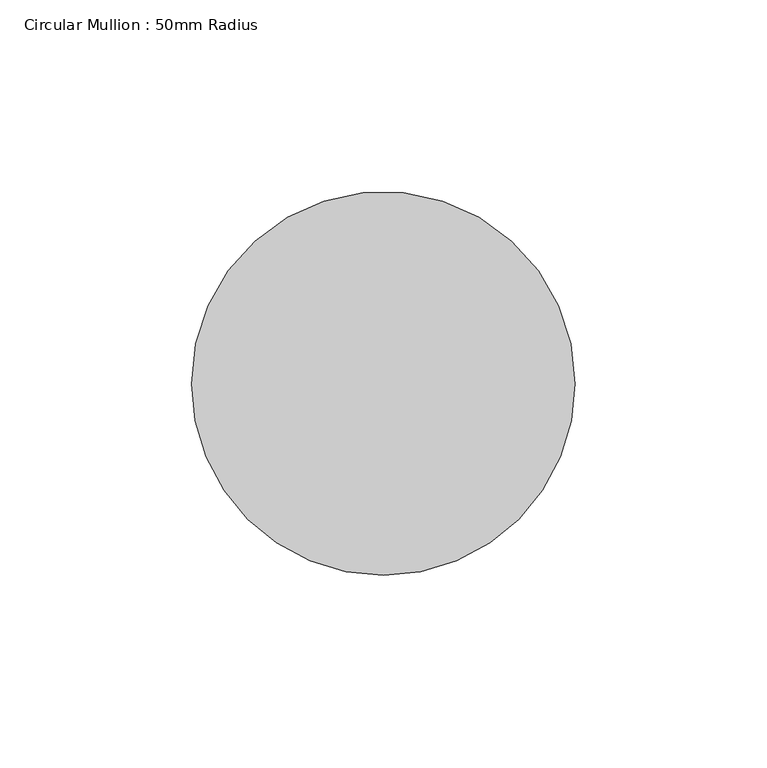
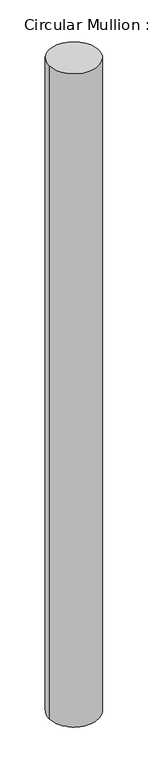
"""IFC4 building model written with IfcOpenShell, lengths in millimetres: member geometry, Circular Mullion : 50mm Radius."""

import ifcopenshell
import ifcopenshell.guid

model = None  # the IFC model being written
_history = None  # IfcOwnerHistory: only IFC2X3 demands one
_inside = {}  # id of a spatial element -> (the spatial element, [elements in it])
_under = {}  # id of a project, library or spatial element -> (it, [spatial elements below it])
_declared = {}  # id of a project -> (the project, [libraries it declares])
_typed = {}  # id of a type object -> (the type object, [elements of that type])
_made_of = {}  # id of a material, layer set ... -> (it, [elements and type objects made of it])


def new_model(schema):
    """Start an empty IFC model of exactly this schema.

    Asked for "IFC4X3", IfcOpenShell would pick the latest addendum, in which some entities
    have other attributes; the version numbers below select the first issue.
    IFC2X3 requires an IfcOwnerHistory on every rooted entity: one is made here for all.
    """
    global model, _history
    if schema == "IFC4X3":
        model = ifcopenshell.file(schema_version=(4, 3, 0, 0))
    else:
        model = ifcopenshell.file(schema=schema)
    _inside.clear()
    _under.clear()
    _declared.clear()
    _typed.clear()
    _made_of.clear()
    _history = None
    if model.schema == "IFC2X3":
        org = make("IfcOrganization", Name="unknown")
        user = make(
            "IfcPersonAndOrganization",
            ThePerson=make("IfcPerson", FamilyName="unknown"),
            TheOrganization=org,
        )
        app = make(
            "IfcApplication",
            ApplicationDeveloper=org,
            Version="unknown",
            ApplicationFullName="unknown",
            ApplicationIdentifier="unknown",
        )
        _history = make(
            "IfcOwnerHistory",
            OwningUser=user,
            OwningApplication=app,
            ChangeAction="ADDED",
            CreationDate=0,
        )
    return model


def make(cls, **values):
    """One entity of the class cls with the attributes given. An attribute that is None is left unset."""
    return model.create_entity(
        cls, **{name: value for name, value in values.items() if value is not None}
    )


def rooted(cls, **values):
    """An entity with a GlobalId (a new one), such as an element, a storey or a relation."""
    return make(cls, GlobalId=ifcopenshell.guid.new(), OwnerHistory=_history, **values)


def si_unit(unit_type, name, prefix=None):
    """IfcSIUnit, for example si_unit("LENGTHUNIT", "METRE", prefix="MILLI")."""
    return make("IfcSIUnit", UnitType=unit_type, Prefix=prefix, Name=name)


def assignment(units):
    """IfcUnitAssignment: the units of a project."""
    return None if units is None else make("IfcUnitAssignment", Units=units)


def point(xyz):
    """IfcCartesianPoint."""
    return None if xyz is None else make("IfcCartesianPoint", Coordinates=xyz)


def direction(xyz):
    """IfcDirection."""
    return None if xyz is None else make("IfcDirection", DirectionRatios=xyz)


def frame(location, z_axis=None, x_axis=None):
    """IfcAxis2Placement3D, a coordinate frame: its origin and axes. An axis left out is left unset."""
    return make(
        "IfcAxis2Placement3D",
        Location=point(location),
        Axis=direction(z_axis),
        RefDirection=direction(x_axis),
    )


def origin():
    """The frame at (0, 0, 0) with its axes left unset."""
    return frame((0.0, 0.0, 0.0))


def place(relative_to, where):
    """IfcLocalPlacement: puts the frame where relative to a parent placement (None: the world)."""
    return make(
        "IfcLocalPlacement", PlacementRelTo=relative_to, RelativePlacement=where
    )


def context(
    kind, dimensions, precision=None, world=None, true_north=None, identifier=None
):
    """IfcGeometricRepresentationContext, for example the 3D "Model" context."""
    return make(
        "IfcGeometricRepresentationContext",
        ContextIdentifier=identifier,
        ContextType=kind,
        CoordinateSpaceDimension=dimensions,
        Precision=precision,
        WorldCoordinateSystem=world,
        TrueNorth=true_north,
    )


def project(units=None, contexts=None):
    """IfcProject with its units and contexts."""
    return rooted(
        "IfcProject",
        Name="project",
        RepresentationContexts=contexts,
        UnitsInContext=assignment(units),
    )


def spatial(cls, under=None, at=None, **own):
    """A site, building, storey or space (cls), placed at a placement, below another one or the project."""
    s = rooted(cls, ObjectPlacement=at, **own)
    if under is not None:
        _under.setdefault(under.id(), (under, []))[1].append(s)
    return s


def ellipse_curve(where, semi_axis1, semi_axis2):
    """IfcEllipse in the frame where."""
    return make(
        "IfcEllipse", Position=where, SemiAxis1=semi_axis1, SemiAxis2=semi_axis2
    )


def shape(context_of_items, identifier, shape_type, items):
    """IfcShapeRepresentation: the items that make up one representation, for example the "Body"."""
    return make(
        "IfcShapeRepresentation",
        ContextOfItems=context_of_items,
        RepresentationIdentifier=identifier,
        RepresentationType=shape_type,
        Items=items,
    )


def source(mapping_origin, context_of_items, identifier, shape_type, items):
    """IfcRepresentationMap: a shape defined once, which mapped items show again and again."""
    return make(
        "IfcRepresentationMap",
        MappingOrigin=mapping_origin,
        MappedRepresentation=shape(context_of_items, identifier, shape_type, items),
    )


def transform(
    local_origin,
    x_axis=None,
    y_axis=None,
    z_axis=None,
    scale=None,
    scale2=None,
    scale3=None,
    uniform=True,
):
    """IfcCartesianTransformationOperator3D, or its non-uniform kind. x_axis, y_axis, z_axis: its Axis1, 2, 3."""
    if uniform:
        return make(
            "IfcCartesianTransformationOperator3D",
            Axis1=direction(x_axis),
            Axis2=direction(y_axis),
            LocalOrigin=point(local_origin),
            Scale=scale,
            Axis3=direction(z_axis),
        )
    return make(
        "IfcCartesianTransformationOperator3DnonUniform",
        Axis1=direction(x_axis),
        Axis2=direction(y_axis),
        LocalOrigin=point(local_origin),
        Scale=scale,
        Axis3=direction(z_axis),
        Scale2=scale2,
        Scale3=scale3,
    )


def mapped(mapping_source, mapping_target):
    """IfcMappedItem: shows the shape of a source again, moved by a transform."""
    return make(
        "IfcMappedItem", MappingSource=mapping_source, MappingTarget=mapping_target
    )


def made_of(thing, what):
    """Note that an element or type object is made of a material, layer set ...; save() writes the relation."""
    if what is not None:
        _made_of.setdefault(what.id(), (what, []))[1].append(thing)
    return thing


def element(
    cls,
    number,
    at=None,
    inside=None,
    cuts=None,
    type_object=None,
    material=None,
    context=None,
    identifier="Body",
    shape_type=None,
    held_by="IfcProductDefinitionShape",
    body=None,
    shapes=None,
    **own,
):
    """One element of the class cls, such as IfcWall. Its Tag is "e" and its number.

    at: its placement. inside: the storey or other place that contains it. cuts: it is an
    opening in that element (IfcRelVoidsElement). A single representation is given by context,
    identifier, shape_type and body (its items); several are given by shapes. held_by: the class
    of the entity that holds the representations. save() writes the other relations.
    """
    e = rooted(cls, Tag="e%d" % number, ObjectPlacement=at, **own)
    if body is not None:
        shapes = [shape(context, identifier, shape_type, body)]
    if shapes is not None:
        e.Representation = make(held_by, Representations=shapes)
    if inside is not None:
        _inside.setdefault(inside.id(), (inside, []))[1].append(e)
    if cuts is not None:
        rooted(
            "IfcRelVoidsElement", RelatingBuildingElement=cuts, RelatedOpeningElement=e
        )
    if type_object is not None:
        _typed.setdefault(type_object.id(), (type_object, []))[1].append(e)
    return made_of(e, material)


def aggregate(whole, parts):
    """IfcRelAggregates: a whole, such as a stair, and the parts it consists of."""
    return rooted("IfcRelAggregates", RelatingObject=whole, RelatedObjects=parts)


def save(model, path):
    """Write the relations noted so far, then the file.

    IfcRelAggregates (storeys below a building ...), IfcRelContainedInSpatialStructure (elements
    in a storey), IfcRelDefinesByType, IfcRelAssociatesMaterial and IfcRelDeclares: one each for
    every whole, place, type object, material and project.
    """
    for whole, parts in _under.values():
        aggregate(whole, parts)
    for where, things in _inside.values():
        rooted(
            "IfcRelContainedInSpatialStructure",
            RelatedElements=things,
            RelatingStructure=where,
        )
    for kind, things in _typed.values():
        rooted("IfcRelDefinesByType", RelatedObjects=things, RelatingType=kind)
    for what, things in _made_of.values():
        rooted("IfcRelAssociatesMaterial", RelatedObjects=things, RelatingMaterial=what)
    for by, libraries in _declared.values():
        rooted("IfcRelDeclares", RelatingContext=by, RelatedDefinitions=libraries)
    model.write(path)


def plane_surface(at):
    """IfcPlane: the flat surface through the origin of the frame at, square to its z axis."""
    return make("IfcPlane", Position=at)


def cylinder_surface(at, radius):
    """IfcCylindricalSurface: all points at the distance radius from the z axis of the frame at."""
    return make("IfcCylindricalSurface", Position=at, Radius=radius)


def advanced_brep(points, edges, surfaces, faces):
    """IfcAdvancedBrep: a solid bounded by faces that lie on surfaces and meet in shared edges.

    An edge is (start, end): straight between two places in points (the first is 0);
    or (start, end, curve); or (start, end, curve, False) where it runs against its curve.
    A face is (place in surfaces, loops), or (place, loops, False) where it looks against
    its surface's normal. A loop lists edges by number (the first is 1), with a minus sign
    where the edge is run from its end to its start. The first loop is the outer one.
    """
    corners = [point(p) for p in points]
    vertices = [make("IfcVertexPoint", VertexGeometry=c) for c in corners]
    made = []
    for start, end, *more in edges:
        made.append(
            make(
                "IfcEdgeCurve",
                EdgeStart=vertices[start],
                EdgeEnd=vertices[end],
                EdgeGeometry=more[0] if more else make("IfcPolyline", Points=[corners[start], corners[end]]),
                SameSense=more[1] if len(more) > 1 else True,
            )
        )
    hull = []
    for where, loops, *sense in faces:
        bounds = []
        for j, loop in enumerate(loops):
            ring = [make("IfcOrientedEdge", EdgeElement=made[abs(k) - 1], Orientation=k > 0) for k in loop]
            bounds.append(
                make(
                    "IfcFaceOuterBound" if j == 0 else "IfcFaceBound",
                    Bound=make("IfcEdgeLoop", EdgeList=ring),
                    Orientation=True,
                )
            )
        hull.append(make("IfcAdvancedFace", Bounds=bounds, FaceSurface=surfaces[where], SameSense=sense[0] if sense else True))
    return make("IfcAdvancedBrep", Outer=make("IfcClosedShell", CfsFaces=hull))


def circular_mullion_50mm_radius_6d670d00(model_context):
    return source(origin(), model_context, "Body", "AdvancedBrep", [
        advanced_brep(
        [(-100.0, 0.0, 0.7566986), (0.0, 0.0, 0.0), (0.0, 0.0, -1386.081394), (-100.0, 0.0, -1386.7912014)],
        [
            (0, 1, ellipse_curve(frame((-50.0, 0.0, 0.3783493), z_axis=(-0.007565809028415525, -0.015931232645763575, -0.9998444650845112), x_axis=(-0.42891947202185954, -0.9031705491658935, 0.017636486040806185)), 50.007778, 50.0)),
            (1, 2),
            (2, 3, ellipse_curve(frame((-50.0, 0.0, -1386.4362977), z_axis=(-0.007097102468351958, -0.014944282906096784, 0.9998631404072141), x_axis=(0.42892748347745896, 0.9031874187911777, 0.016543894796071792)), 50.0068439, 50.0)),
            (3, 0),
            (1, 0, ellipse_curve(frame((-50.0, 0.0, 0.3783493), z_axis=(-0.007565809028415525, -0.015931232645763575, -0.9998444650845112), x_axis=(-0.42891947202185954, -0.9031705491658935, 0.017636486040806185)), 50.007778, 50.0)),
            (3, 2, ellipse_curve(frame((-50.0, 0.0, -1386.4362977), z_axis=(-0.007097102468351958, -0.014944282906096784, 0.9998631404072141), x_axis=(0.42892748347745896, 0.9031874187911777, 0.016543894796071792)), 50.0068439, 50.0)),
        ],
        [
            cylinder_surface(frame((-50.0, 0.0, 0.0), z_axis=(0.0, 0.0, 1.0), x_axis=(1.0, 0.0, 0.0)), 50.0),
            plane_surface(frame((-275.3292067, 130.754992, 0.0), z_axis=(0.007565809028415525, 0.015931232645763575, 0.9998444650845112), x_axis=(0.4289194720218597, 0.9031705491658933, -0.01763648604081598))),
            plane_surface(frame((-275.3292067, 130.754992, -1386.081394), z_axis=(0.007097102468351958, 0.014944282906096784, -0.9998631404072141), x_axis=(0.42892748347745907, 0.9031874187911778, 0.016543894796079428))),
        ],
        [
            (0, [[1, 2, 3, 4]]),
            (0, [[5, -4, 6, -2]]),
            (1, [[-1, -5]]),
            (2, [[-6, -3]]),
        ],
    ),
    ])


if __name__ == "__main__":
    model = new_model("IFC4")
    model_context = context("Model", 3, world=origin())
    ifc_project = project(units=[si_unit("LENGTHUNIT", "METRE", prefix="MILLI")], contexts=[model_context])
    site = spatial("IfcSite", under=ifc_project)
    building = spatial("IfcBuilding", under=site)
    placement = place(None, origin())
    circular_mullion_50mm_radius_shape = circular_mullion_50mm_radius_6d670d00(model_context)
    element("IfcMember", 1, ObjectType="Circular Mullion : 50mm Radius", at=placement, inside=building, context=model_context, shape_type="MappedRepresentation", body=[
        mapped(circular_mullion_50mm_radius_shape, transform((0.0, 0.0, 0.0), x_axis=(1.0, 0.0, 0.0), y_axis=(0.0, 1.0, 0.0), z_axis=(0.0, 0.0, 1.0))),
    ])
    save(model, "model.ifc")

# Revit data of these elements
# Type "Circular Mullion : 50mm Radius"
#   built-in parameter 1007350 = 0.164042 (stored number, unit not read)
# Element 1 (IfcMember, "Circular Mullion : 50mm Radius")
#   Materials on its faces: "Aluminium"
# Materials
#   "Aluminium": class "Metal", colour RGB 247 247 247, transparency 0, Description = "Aluminium 6061", Cost = 0
